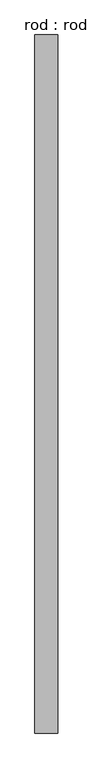
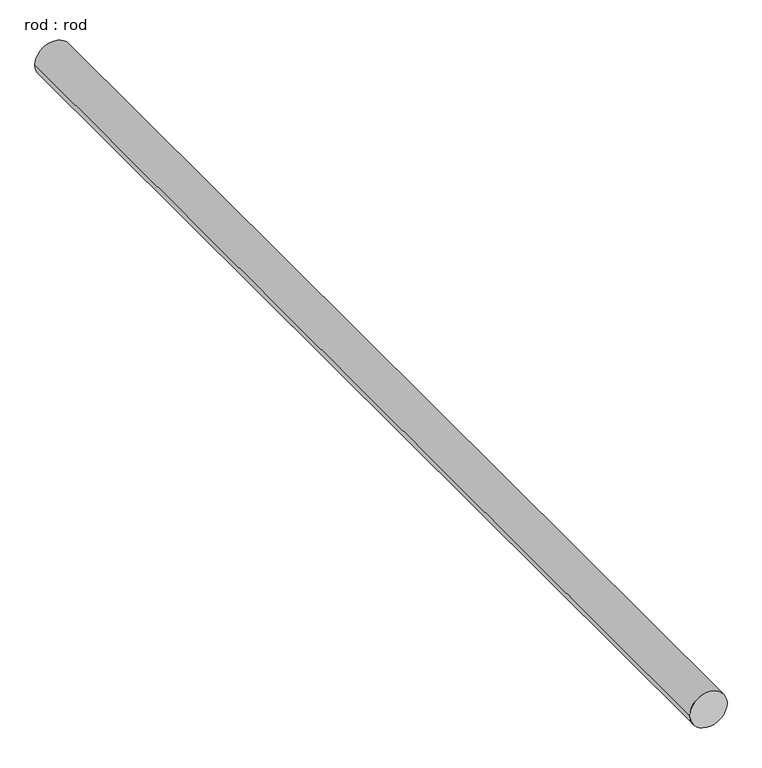
"""IFC4 building model written with IfcOpenShell, lengths in millimetres: proxy geometry, rod : rod."""

import ifcopenshell
import ifcopenshell.guid

model = None  # the IFC model being written
_history = None  # IfcOwnerHistory: only IFC2X3 demands one
_inside = {}  # id of a spatial element -> (the spatial element, [elements in it])
_under = {}  # id of a project, library or spatial element -> (it, [spatial elements below it])
_declared = {}  # id of a project -> (the project, [libraries it declares])
_typed = {}  # id of a type object -> (the type object, [elements of that type])
_made_of = {}  # id of a material, layer set ... -> (it, [elements and type objects made of it])


def new_model(schema):
    """Start an empty IFC model of exactly this schema.

    Asked for "IFC4X3", IfcOpenShell would pick the latest addendum, in which some entities
    have other attributes; the version numbers below select the first issue.
    IFC2X3 requires an IfcOwnerHistory on every rooted entity: one is made here for all.
    """
    global model, _history
    if schema == "IFC4X3":
        model = ifcopenshell.file(schema_version=(4, 3, 0, 0))
    else:
        model = ifcopenshell.file(schema=schema)
    _inside.clear()
    _under.clear()
    _declared.clear()
    _typed.clear()
    _made_of.clear()
    _history = None
    if model.schema == "IFC2X3":
        org = make("IfcOrganization", Name="unknown")
        user = make(
            "IfcPersonAndOrganization",
            ThePerson=make("IfcPerson", FamilyName="unknown"),
            TheOrganization=org,
        )
        app = make(
            "IfcApplication",
            ApplicationDeveloper=org,
            Version="unknown",
            ApplicationFullName="unknown",
            ApplicationIdentifier="unknown",
        )
        _history = make(
            "IfcOwnerHistory",
            OwningUser=user,
            OwningApplication=app,
            ChangeAction="ADDED",
            CreationDate=0,
        )
    return model


def make(cls, **values):
    """One entity of the class cls with the attributes given. An attribute that is None is left unset."""
    return model.create_entity(
        cls, **{name: value for name, value in values.items() if value is not None}
    )


def rooted(cls, **values):
    """An entity with a GlobalId (a new one), such as an element, a storey or a relation."""
    return make(cls, GlobalId=ifcopenshell.guid.new(), OwnerHistory=_history, **values)


def si_unit(unit_type, name, prefix=None):
    """IfcSIUnit, for example si_unit("LENGTHUNIT", "METRE", prefix="MILLI")."""
    return make("IfcSIUnit", UnitType=unit_type, Prefix=prefix, Name=name)


def assignment(units):
    """IfcUnitAssignment: the units of a project."""
    return None if units is None else make("IfcUnitAssignment", Units=units)


def point(xyz):
    """IfcCartesianPoint."""
    return None if xyz is None else make("IfcCartesianPoint", Coordinates=xyz)


def direction(xyz):
    """IfcDirection."""
    return None if xyz is None else make("IfcDirection", DirectionRatios=xyz)


def frame(location, z_axis=None, x_axis=None):
    """IfcAxis2Placement3D, a coordinate frame: its origin and axes. An axis left out is left unset."""
    return make(
        "IfcAxis2Placement3D",
        Location=point(location),
        Axis=direction(z_axis),
        RefDirection=direction(x_axis),
    )


def frame_2d(location, x_axis=None):
    """IfcAxis2Placement2D, a coordinate frame in the plane: its origin and x axis."""
    return make(
        "IfcAxis2Placement2D", Location=point(location), RefDirection=direction(x_axis)
    )


def origin():
    """The frame at (0, 0, 0) with its axes left unset."""
    return frame((0.0, 0.0, 0.0))


def place(relative_to, where):
    """IfcLocalPlacement: puts the frame where relative to a parent placement (None: the world)."""
    return make(
        "IfcLocalPlacement", PlacementRelTo=relative_to, RelativePlacement=where
    )


def context(
    kind, dimensions, precision=None, world=None, true_north=None, identifier=None
):
    """IfcGeometricRepresentationContext, for example the 3D "Model" context."""
    return make(
        "IfcGeometricRepresentationContext",
        ContextIdentifier=identifier,
        ContextType=kind,
        CoordinateSpaceDimension=dimensions,
        Precision=precision,
        WorldCoordinateSystem=world,
        TrueNorth=true_north,
    )


def project(units=None, contexts=None):
    """IfcProject with its units and contexts."""
    return rooted(
        "IfcProject",
        Name="project",
        RepresentationContexts=contexts,
        UnitsInContext=assignment(units),
    )


def spatial(cls, under=None, at=None, **own):
    """A site, building, storey or space (cls), placed at a placement, below another one or the project."""
    s = rooted(cls, ObjectPlacement=at, **own)
    if under is not None:
        _under.setdefault(under.id(), (under, []))[1].append(s)
    return s


def circle_curve(where, radius):
    """IfcCircle in the frame where."""
    return make("IfcCircle", Position=where, Radius=radius)


def trimmed(basis, trim1, trim2, sense, master):
    """IfcTrimmedCurve: the piece of a basis curve between two trims."""
    return make(
        "IfcTrimmedCurve",
        BasisCurve=basis,
        Trim1=trim1,
        Trim2=trim2,
        SenseAgreement=sense,
        MasterRepresentation=master,
    )


def segment(curve, same_sense, transition):
    """IfcCompositeCurveSegment."""
    return make(
        "IfcCompositeCurveSegment",
        Transition=transition,
        SameSense=same_sense,
        ParentCurve=curve,
    )


def composite_curve(segments, self_intersect=None):
    """IfcCompositeCurve: segments joined end to end."""
    return make("IfcCompositeCurve", Segments=segments, SelfIntersect=self_intersect)


def outline(outer, holes=None, kind="AREA"):
    """IfcArbitraryClosedProfileDef: a profile drawn as a closed curve; with holes, ...WithVoids."""
    if holes is None:
        return make("IfcArbitraryClosedProfileDef", ProfileType=kind, OuterCurve=outer)
    return make(
        "IfcArbitraryProfileDefWithVoids",
        ProfileType=kind,
        OuterCurve=outer,
        InnerCurves=holes,
    )


def extrude(swept, where, along, depth):
    """IfcExtrudedAreaSolid: the profile swept, set in the frame where, extruded along a direction by depth."""
    return make(
        "IfcExtrudedAreaSolid",
        SweptArea=swept,
        Position=where,
        ExtrudedDirection=direction(along),
        Depth=depth,
    )


def shape(context_of_items, identifier, shape_type, items):
    """IfcShapeRepresentation: the items that make up one representation, for example the "Body"."""
    return make(
        "IfcShapeRepresentation",
        ContextOfItems=context_of_items,
        RepresentationIdentifier=identifier,
        RepresentationType=shape_type,
        Items=items,
    )


def source(mapping_origin, context_of_items, identifier, shape_type, items):
    """IfcRepresentationMap: a shape defined once, which mapped items show again and again."""
    return make(
        "IfcRepresentationMap",
        MappingOrigin=mapping_origin,
        MappedRepresentation=shape(context_of_items, identifier, shape_type, items),
    )


def transform(
    local_origin,
    x_axis=None,
    y_axis=None,
    z_axis=None,
    scale=None,
    scale2=None,
    scale3=None,
    uniform=True,
):
    """IfcCartesianTransformationOperator3D, or its non-uniform kind. x_axis, y_axis, z_axis: its Axis1, 2, 3."""
    if uniform:
        return make(
            "IfcCartesianTransformationOperator3D",
            Axis1=direction(x_axis),
            Axis2=direction(y_axis),
            LocalOrigin=point(local_origin),
            Scale=scale,
            Axis3=direction(z_axis),
        )
    return make(
        "IfcCartesianTransformationOperator3DnonUniform",
        Axis1=direction(x_axis),
        Axis2=direction(y_axis),
        LocalOrigin=point(local_origin),
        Scale=scale,
        Axis3=direction(z_axis),
        Scale2=scale2,
        Scale3=scale3,
    )


def mapped(mapping_source, mapping_target):
    """IfcMappedItem: shows the shape of a source again, moved by a transform."""
    return make(
        "IfcMappedItem", MappingSource=mapping_source, MappingTarget=mapping_target
    )


def made_of(thing, what):
    """Note that an element or type object is made of a material, layer set ...; save() writes the relation."""
    if what is not None:
        _made_of.setdefault(what.id(), (what, []))[1].append(thing)
    return thing


def element(
    cls,
    number,
    at=None,
    inside=None,
    cuts=None,
    type_object=None,
    material=None,
    context=None,
    identifier="Body",
    shape_type=None,
    held_by="IfcProductDefinitionShape",
    body=None,
    shapes=None,
    **own,
):
    """One element of the class cls, such as IfcWall. Its Tag is "e" and its number.

    at: its placement. inside: the storey or other place that contains it. cuts: it is an
    opening in that element (IfcRelVoidsElement). A single representation is given by context,
    identifier, shape_type and body (its items); several are given by shapes. held_by: the class
    of the entity that holds the representations. save() writes the other relations.
    """
    e = rooted(cls, Tag="e%d" % number, ObjectPlacement=at, **own)
    if body is not None:
        shapes = [shape(context, identifier, shape_type, body)]
    if shapes is not None:
        e.Representation = make(held_by, Representations=shapes)
    if inside is not None:
        _inside.setdefault(inside.id(), (inside, []))[1].append(e)
    if cuts is not None:
        rooted(
            "IfcRelVoidsElement", RelatingBuildingElement=cuts, RelatedOpeningElement=e
        )
    if type_object is not None:
        _typed.setdefault(type_object.id(), (type_object, []))[1].append(e)
    return made_of(e, material)


def aggregate(whole, parts):
    """IfcRelAggregates: a whole, such as a stair, and the parts it consists of."""
    return rooted("IfcRelAggregates", RelatingObject=whole, RelatedObjects=parts)


def save(model, path):
    """Write the relations noted so far, then the file.

    IfcRelAggregates (storeys below a building ...), IfcRelContainedInSpatialStructure (elements
    in a storey), IfcRelDefinesByType, IfcRelAssociatesMaterial and IfcRelDeclares: one each for
    every whole, place, type object, material and project.
    """
    for whole, parts in _under.values():
        aggregate(whole, parts)
    for where, things in _inside.values():
        rooted(
            "IfcRelContainedInSpatialStructure",
            RelatedElements=things,
            RelatingStructure=where,
        )
    for kind, things in _typed.values():
        rooted("IfcRelDefinesByType", RelatedObjects=things, RelatingType=kind)
    for what, things in _made_of.values():
        rooted("IfcRelAssociatesMaterial", RelatedObjects=things, RelatingMaterial=what)
    for by, libraries in _declared.values():
        rooted("IfcRelDeclares", RelatingContext=by, RelatedDefinitions=libraries)
    model.write(path)


def rod_rod_dd8d50f1(model_context):
    return source(origin(), model_context, "Body", "SweptSolid", [
        extrude(outline(composite_curve([segment(trimmed(circle_curve(frame_2d((0.0108462, 0.0)), 200.0), [point((0.0108462, 200.0))], [point((0.0108462, -200.0))], False, "CARTESIAN"), True, "CONTINUOUS"), segment(trimmed(circle_curve(frame_2d((0.0108462, 0.0)), 200.0), [point((0.0108462, -200.0))], [point((0.0108462, 200.0))], False, "CARTESIAN"), True, "CONTINUOUS")], self_intersect=False)), frame((0.0, -2007.2713847, 0.0), z_axis=(0.0, 1.0, 0.0), x_axis=(0.0, 0.0, 1.0)), (0.0, 0.0, 1.0), 12200.0),
    ])


if __name__ == "__main__":
    model = new_model("IFC4")
    model_context = context("Model", 3, world=origin())
    ifc_project = project(units=[si_unit("LENGTHUNIT", "METRE", prefix="MILLI")], contexts=[model_context])
    site = spatial("IfcSite", under=ifc_project)
    building = spatial("IfcBuilding", under=site)
    placement = place(None, origin())
    rod_rod_shape = rod_rod_dd8d50f1(model_context)
    element("IfcBuildingElementProxy", 1, Name="rod : rod", ObjectType="rod : rod", at=placement, inside=building, context=model_context, shape_type="MappedRepresentation", body=[
        mapped(rod_rod_shape, transform((0.0, 0.0, 0.0), x_axis=(1.0, 0.0, 0.0), y_axis=(0.0, 1.0, 0.0), z_axis=(0.0, 0.0, 1.0))),
    ])
    save(model, "model.ifc")

# Revit data of these elements
# Type "rod : rod"
#   Default Elevation = 0
